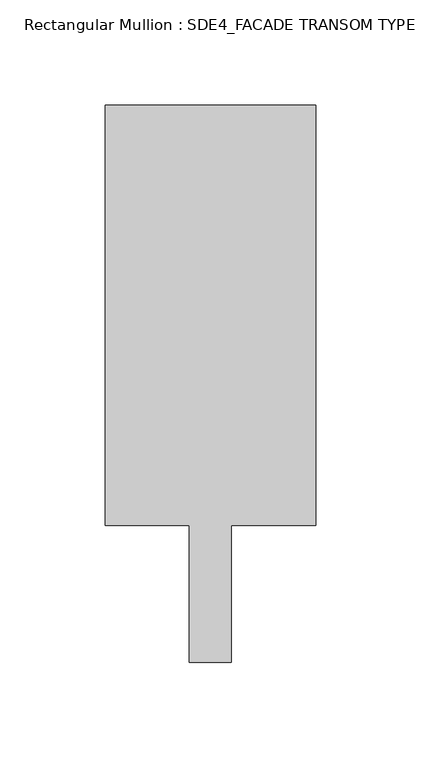
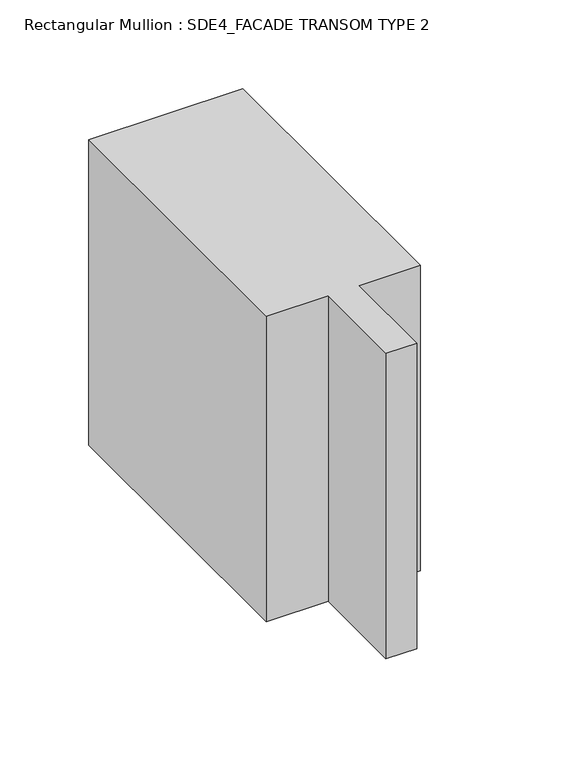
"""IFC4 building model written with IfcOpenShell, lengths in millimetres: member geometry, Rectangular Mullion : SDE4_FACADE TRANSOM TYPE 2."""

from ifc_helpers import new_model, si_unit, frame, origin, place, context, project, spatial, polyline, outline, extrude, source, transform, mapped, element, save


def rectangular_mullion_sde4_facade_transom_type_2_1f5b38cd(model_context):
    return source(origin(), model_context, "Body", "SweptSolid", [
        extrude(outline(polyline([(50.0, 132.5), (50.0, -67.5), (10.0, -67.5), (10.0, -132.5), (-10.0, -132.5), (-10.0, -67.5), (-50.0, -67.5), (-50.0, 132.5), (50.0, 132.5)])), frame((0.0, 0.0, -209.9239219), z_axis=(0.0, 0.0, 1.0), x_axis=(1.0, 0.0, 0.0)), (0.0, 0.0, 1.0), 209.9239219),
    ])


if __name__ == "__main__":
    model = new_model("IFC4")
    model_context = context("Model", 3, world=origin())
    ifc_project = project(units=[si_unit("LENGTHUNIT", "METRE", prefix="MILLI")], contexts=[model_context])
    site = spatial("IfcSite", under=ifc_project)
    building = spatial("IfcBuilding", under=site)
    placement = place(None, origin())
    rectangular_mullion_sde4_facade_transom_type_2_shape = rectangular_mullion_sde4_facade_transom_type_2_1f5b38cd(model_context)
    element("IfcMember", 1, ObjectType="Rectangular Mullion : SDE4_FACADE TRANSOM TYPE 2", at=placement, inside=building, context=model_context, shape_type="MappedRepresentation", body=[
        mapped(rectangular_mullion_sde4_facade_transom_type_2_shape, transform((0.0, 0.0, 0.0), x_axis=(1.0, 0.0, 0.0), y_axis=(0.0, 1.0, 0.0), z_axis=(0.0, 0.0, 1.0))),
    ])
    save(model, "model.ifc")

# Revit data of these elements
# Type "Rectangular Mullion : SDE4_FACADE TRANSOM TYPE 2"
#   built-in parameter 1007322 = 0.869423 (stored number, unit not read)
#   built-in parameter 1007321 = 0.164042 (stored number, unit not read)
#   built-in parameter 1007320 = 0.164042 (stored number, unit not read)
